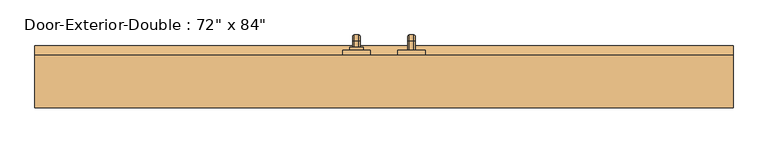
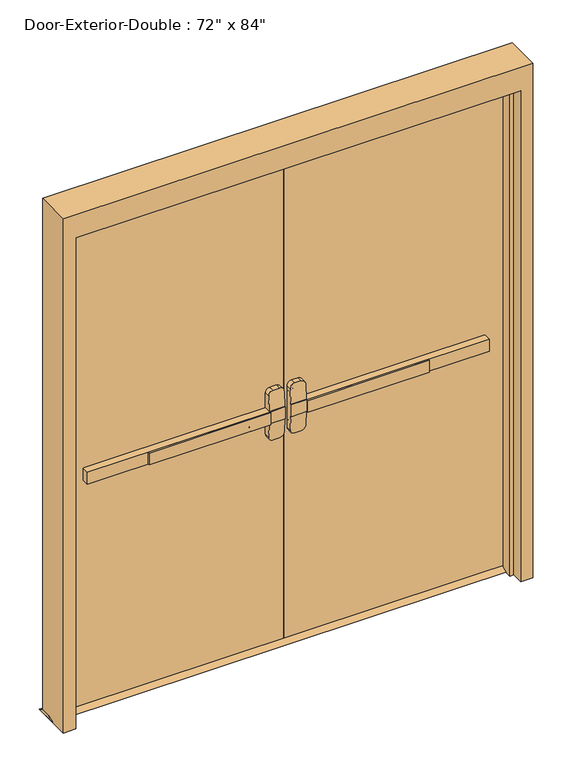
"""IFC4 building model written with IfcOpenShell, lengths in millimetres: door geometry."""

from ifc_helpers import new_model, si_unit, point, frame, frame_2d, origin, place, context, project, spatial, polyline, circle_curve, ellipse_curve, trimmed, segment, composite_curve, outline, extrude, faceted_brep, source, transform, mapped, element, save
from ifc_brep_helpers import plane_surface, cylinder_surface, revolved_surface, advanced_brep


def door_9c6f9228(model_context):
    return source(origin(), model_context, "Body", "SolidModel", [
        extrude(outline(polyline([(-575.7333333, -3.175), (-575.7333333, 3.175), (-76.2, 3.175), (-76.2, -3.175), (-575.7333333, -3.175)])), frame((0.0, 0.0, 990.6), z_axis=(0.0, 0.0, 1.0), x_axis=(1.0, 0.0, 0.0)), (0.0, 0.0, 1.0), 50.8),
        advanced_brep(
        [(-12.7, 3.175, 1041.4), (-76.2, 3.175, 1041.4), (-825.5, 3.175, 1041.4), (-825.5, 3.175, 990.6), (-76.2, 3.175, 990.6), (-12.7, 3.175, 990.6), (-825.5, 34.925, 1041.4), (-76.2, 34.925, 1041.4), (-76.2, 34.925, 1104.9), (-57.15, 34.925, 1123.95), (-31.75, 34.925, 1123.95), (-12.7, 34.925, 1104.9), (-12.7, 34.925, 927.1), (-31.75, 34.925, 908.05), (-57.15, 34.925, 908.05), (-76.2, 34.925, 927.1), (-76.2, 34.925, 990.6), (-825.5, 34.925, 990.6), (-12.7, 6.3502467, 1041.4), (-76.2, 6.3502467, 1041.4), (-12.7, 6.3502467, 990.6), (-12.7, 11.3604269, 927.1), (-12.7, 11.3604269, 1104.9), (-76.2, 6.3502467, 990.6), (-76.2, 11.3604269, 1104.9), (-76.2, 11.3604269, 927.1), (-57.15, 12.863481, 1123.95), (-31.75, 12.863481, 1123.95), (-31.75, 12.863481, 908.05), (-57.15, 12.863481, 908.05)],
        [
            (0, 1),
            (1, 2),
            (2, 3),
            (3, 4),
            (4, 5),
            (5, 0),
            (6, 7),
            (7, 8),
            (8, 9, circle_curve(frame((-57.15, 34.925, 1104.9), z_axis=(0.0, 1.0, 0.0), x_axis=(-1.0, 0.0, 0.0)), 19.05)),
            (9, 10),
            (10, 11, circle_curve(frame((-31.75, 34.925, 1104.9), z_axis=(0.0, 1.0, 0.0), x_axis=(-1.0, 0.0, 0.0)), 19.05)),
            (11, 12),
            (12, 13, circle_curve(frame((-31.75, 34.925, 927.1), z_axis=(0.0, 1.0, 0.0), x_axis=(-1.0, 0.0, 0.0)), 19.05)),
            (13, 14),
            (14, 15, circle_curve(frame((-57.15, 34.925, 927.1), z_axis=(0.0, 1.0, 0.0), x_axis=(-1.0, 0.0, 0.0)), 19.05)),
            (15, 16),
            (16, 17),
            (17, 6),
            (0, 18),
            (18, 19),
            (19, 7),
            (6, 2),
            (5, 20),
            (20, 21),
            (21, 12),
            (11, 22),
            (22, 18),
            (16, 23),
            (23, 20),
            (3, 17),
            (19, 24),
            (24, 8),
            (15, 25),
            (25, 23),
            (9, 26),
            (26, 27),
            (27, 10),
            (13, 28),
            (28, 29),
            (29, 14),
            (29, 25, ellipse_curve(frame((-57.15, 11.3604269, 927.1), z_axis=(0.0, 0.9969018152893365, 0.07865602756830282), x_axis=(0.0, -0.07865602756830208, 0.9969018152893365)), 19.1092038, 19.05)),
            (24, 26, ellipse_curve(frame((-57.15, 11.3604269, 1104.9), z_axis=(0.0, 0.9969018152893376, -0.07865602756828934), x_axis=(0.0, -0.078656027568288, -0.9969018152893377)), 19.1092038, 19.05)),
            (27, 22, ellipse_curve(frame((-31.75, 11.3604269, 1104.9), z_axis=(0.0, 0.9969018152893376, -0.07865602756828934), x_axis=(0.0, -0.078656027568288, -0.9969018152893377)), 19.1092038, 19.05)),
            (21, 28, ellipse_curve(frame((-31.75, 11.3604269, 927.1), z_axis=(0.0, 0.9969018152893365, 0.07865602756830282), x_axis=(0.0, -0.07865602756830208, 0.9969018152893365)), 19.1092038, 19.05)),
        ],
        [
            plane_surface(frame((-12.7, 3.175, 1041.4), z_axis=(0.0, -1.0, 0.0), x_axis=(1.0, 0.0, 0.0))),
            plane_surface(frame((-12.7, 34.925, 1041.4), z_axis=(0.0, 1.0, 0.0), x_axis=(-1.0, 0.0, 0.0))),
            plane_surface(frame((-825.5, 3.175, 1041.4), z_axis=(0.0, 0.0, 1.0), x_axis=(0.0, 1.0, 0.0))),
            plane_surface(frame((-12.7, 3.175, 1041.4), z_axis=(1.0, 0.0, 0.0), x_axis=(0.0, 1.0, 0.0))),
            plane_surface(frame((-12.7, 3.175, 990.6), z_axis=(0.0, 0.0, -1.0), x_axis=(0.0, 1.0, 0.0))),
            plane_surface(frame((-825.5, 3.175, 990.6), z_axis=(-1.0, 0.0, 0.0), x_axis=(0.0, 1.0, 0.0))),
            plane_surface(frame((-76.2, 6.3502467, 927.1), z_axis=(-1.0, 0.0, 0.0), x_axis=(0.0, 1.0, 0.0))),
            plane_surface(frame((-57.15, 6.3502467, 1123.95), z_axis=(0.0, 0.0, 1.0), x_axis=(0.0, 1.0, 0.0))),
            plane_surface(frame((-31.75, 6.3502467, 908.05), z_axis=(0.0, 0.0, -1.0), x_axis=(0.0, 1.0, 0.0))),
            cylinder_surface(frame((-57.15, 34.925, 927.1), z_axis=(0.0, -1.0, 0.0), x_axis=(-1.0, 0.0, 0.0)), 19.05),
            cylinder_surface(frame((-57.15, 34.925, 1104.9), z_axis=(0.0, -1.0, 0.0), x_axis=(-1.0, 0.0, 0.0)), 19.05),
            cylinder_surface(frame((-31.75, 34.925, 1104.9), z_axis=(0.0, -1.0, 0.0), x_axis=(-1.0, 0.0, 0.0)), 19.05),
            cylinder_surface(frame((-31.75, 34.925, 927.1), z_axis=(0.0, -1.0, 0.0), x_axis=(-1.0, 0.0, 0.0)), 19.05),
            plane_surface(frame((-76.2, 6.3502467, 1041.4), z_axis=(0.0, -0.9969018152893376, 0.07865602756828934), x_axis=(1.0, 0.0, 0.0))),
            plane_surface(frame((-76.2, 12.863481, 908.05), z_axis=(0.0, -0.9969018152893365, -0.07865602756830282), x_axis=(1.0, 0.0, 0.0))),
        ],
        [
            (0, [[1, 2, 3, 4, 5, 6]]),
            (1, [[7, 8, 9, 10, 11, 12, 13, 14, 15, 16, 17, 18]]),
            (2, [[-2, -1, 19, 20, 21, -7, 22]]),
            (3, [[23, 24, 25, -12, 26, 27, -19, -6]]),
            (4, [[-17, 28, 29, -23, -5, -4, 30]]),
            (5, [[-22, -18, -30, -3]]),
            (6, [[-21, 31, 32, -8]]),
            (6, [[33, 34, -28, -16]]),
            (7, [[35, 36, 37, -10]]),
            (8, [[38, 39, 40, -14]]),
            (9, [[-40, 41, -33, -15]]),
            (10, [[-32, 42, -35, -9]]),
            (11, [[-37, 43, -26, -11]]),
            (12, [[-25, 44, -38, -13]]),
            (13, [[-27, -43, -36, -42, -31, -20]]),
            (14, [[-29, -34, -41, -39, -44, -24]]),
        ],
    ),
        extrude(outline(polyline([(79.375, 12.7), (104.775, 0.0), (9.525, 0.0), (34.925, 12.7), (79.375, 12.7)])), frame((-965.2, 0.0, 0.0), z_axis=(1.0, 0.0, 0.0), x_axis=(0.0, 1.0, 0.0)), (0.0, 0.0, 1.0), 1930.4),
        extrude(outline(polyline([(575.7333333, -3.175), (76.2, -3.175), (76.2, 3.175), (575.7333333, 3.175), (575.7333333, -3.175)])), frame((0.0, 0.0, 990.6), z_axis=(0.0, 0.0, 1.0), x_axis=(1.0, 0.0, 0.0)), (0.0, 0.0, 1.0), 50.8),
        advanced_brep(
        [(12.7, 3.175, 1041.4), (12.7, 3.175, 990.6), (76.2, 3.175, 990.6), (825.5, 3.175, 990.6), (825.5, 3.175, 1041.4), (76.2, 3.175, 1041.4), (825.5, 34.925, 1041.4), (825.5, 34.925, 990.6), (76.2, 34.925, 990.6), (76.2, 34.925, 927.1), (57.15, 34.925, 908.05), (31.75, 34.925, 908.05), (12.7, 34.925, 927.1), (12.7, 34.925, 1104.9), (31.75, 34.925, 1123.95), (57.15, 34.925, 1123.95), (76.2, 34.925, 1104.9), (76.2, 34.925, 1041.4), (76.2, 6.3502467, 1041.4), (12.7, 6.3502467, 1041.4), (12.7, 11.3604269, 1104.9), (12.7, 11.3604269, 927.1), (12.7, 6.3502467, 990.6), (76.2, 6.3502467, 990.6), (76.2, 11.3604269, 927.1), (76.2, 11.3604269, 1104.9), (31.75, 12.863481, 1123.95), (57.15, 12.863481, 1123.95), (57.15, 12.863481, 908.05), (31.75, 12.863481, 908.05)],
        [
            (0, 1),
            (1, 2),
            (2, 3),
            (3, 4),
            (4, 5),
            (5, 0),
            (6, 7),
            (7, 8),
            (8, 9),
            (9, 10, circle_curve(frame((57.15, 34.925, 927.1), z_axis=(0.0, 1.0, 0.0), x_axis=(1.0, 0.0, 0.0)), 19.05)),
            (10, 11),
            (11, 12, circle_curve(frame((31.75, 34.925, 927.1), z_axis=(0.0, 1.0, 0.0), x_axis=(1.0, 0.0, 0.0)), 19.05)),
            (12, 13),
            (13, 14, circle_curve(frame((31.75, 34.925, 1104.9), z_axis=(0.0, 1.0, 0.0), x_axis=(1.0, 0.0, 0.0)), 19.05)),
            (14, 15),
            (15, 16, circle_curve(frame((57.15, 34.925, 1104.9), z_axis=(0.0, 1.0, 0.0), x_axis=(1.0, 0.0, 0.0)), 19.05)),
            (16, 17),
            (17, 6),
            (4, 6),
            (17, 18),
            (18, 19),
            (19, 0),
            (19, 20),
            (20, 13),
            (12, 21),
            (21, 22),
            (22, 1),
            (7, 3),
            (22, 23),
            (23, 8),
            (23, 24),
            (24, 9),
            (16, 25),
            (25, 18),
            (14, 26),
            (26, 27),
            (27, 15),
            (10, 28),
            (28, 29),
            (29, 11),
            (24, 28, ellipse_curve(frame((57.15, 11.3604269, 927.1), z_axis=(0.0, 0.9969018152893365, 0.07865602756830282), x_axis=(0.0, -0.07865602756830208, 0.9969018152893365)), 19.1092038, 19.05)),
            (27, 25, ellipse_curve(frame((57.15, 11.3604269, 1104.9), z_axis=(0.0, 0.9969018152893376, -0.07865602756828934), x_axis=(0.0, -0.078656027568288, -0.9969018152893377)), 19.1092038, 19.05)),
            (20, 26, ellipse_curve(frame((31.75, 11.3604269, 1104.9), z_axis=(0.0, 0.9969018152893376, -0.07865602756828934), x_axis=(0.0, -0.078656027568288, -0.9969018152893377)), 19.1092038, 19.05)),
            (29, 21, ellipse_curve(frame((31.75, 11.3604269, 927.1), z_axis=(0.0, 0.9969018152893365, 0.07865602756830282), x_axis=(0.0, -0.07865602756830208, 0.9969018152893365)), 19.1092038, 19.05)),
        ],
        [
            plane_surface(frame((12.7, 3.175, 1041.4), z_axis=(0.0, -1.0, 0.0), x_axis=(-1.0, 0.0, 0.0))),
            plane_surface(frame((12.7, 34.925, 1041.4), z_axis=(0.0, 1.0, 0.0), x_axis=(1.0, 0.0, 0.0))),
            plane_surface(frame((825.5, 3.175, 1041.4), z_axis=(0.0, 0.0, 1.0), x_axis=(0.0, 1.0, 0.0))),
            plane_surface(frame((12.7, 3.175, 1041.4), z_axis=(-1.0, 0.0, 0.0), x_axis=(0.0, 1.0, 0.0))),
            plane_surface(frame((12.7, 3.175, 990.6), z_axis=(0.0, 0.0, -1.0), x_axis=(0.0, 1.0, 0.0))),
            plane_surface(frame((825.5, 3.175, 990.6), z_axis=(1.0, 0.0, 0.0), x_axis=(0.0, 1.0, 0.0))),
            plane_surface(frame((76.2, 6.3502467, 927.1), z_axis=(1.0, 0.0, 0.0), x_axis=(0.0, 1.0, 0.0))),
            plane_surface(frame((57.15, 6.3502467, 1123.95), z_axis=(0.0, 0.0, 1.0), x_axis=(0.0, 1.0, 0.0))),
            plane_surface(frame((31.75, 6.3502467, 908.05), z_axis=(0.0, 0.0, -1.0), x_axis=(0.0, 1.0, 0.0))),
            cylinder_surface(frame((57.15, 34.925, 927.1), z_axis=(0.0, -1.0, 0.0), x_axis=(1.0, 0.0, 0.0)), 19.05),
            cylinder_surface(frame((57.15, 34.925, 1104.9), z_axis=(0.0, -1.0, 0.0), x_axis=(1.0, 0.0, 0.0)), 19.05),
            cylinder_surface(frame((31.75, 34.925, 1104.9), z_axis=(0.0, -1.0, 0.0), x_axis=(1.0, 0.0, 0.0)), 19.05),
            cylinder_surface(frame((31.75, 34.925, 927.1), z_axis=(0.0, -1.0, 0.0), x_axis=(1.0, 0.0, 0.0)), 19.05),
            plane_surface(frame((76.2, 6.3502467, 1041.4), z_axis=(0.0, -0.9969018152893376, 0.07865602756828934), x_axis=(-1.0, 0.0, 0.0))),
            plane_surface(frame((76.2, 12.863481, 908.05), z_axis=(0.0, -0.9969018152893365, -0.07865602756830282), x_axis=(-1.0, 0.0, 0.0))),
        ],
        [
            (0, [[1, 2, 3, 4, 5, 6]]),
            (1, [[7, 8, 9, 10, 11, 12, 13, 14, 15, 16, 17, 18]]),
            (2, [[19, -18, 20, 21, 22, -6, -5]]),
            (3, [[-1, -22, 23, 24, -13, 25, 26, 27]]),
            (4, [[28, -3, -2, -27, 29, 30, -8]]),
            (5, [[-4, -28, -7, -19]]),
            (6, [[-9, -30, 31, 32]]),
            (6, [[-17, 33, 34, -20]]),
            (7, [[-15, 35, 36, 37]]),
            (8, [[-11, 38, 39, 40]]),
            (9, [[-10, -32, 41, -38]]),
            (10, [[-16, -37, 42, -33]]),
            (11, [[-14, -24, 43, -35]]),
            (12, [[-12, -40, 44, -25]]),
            (13, [[-21, -34, -42, -36, -43, -23]]),
            (14, [[-26, -44, -39, -41, -31, -29]]),
        ],
    ),
        advanced_brep(
        [(66.2, 92.075, 1017.190625), (66.2, 92.075, 1014.809375), (69.771875, 92.075, 1011.2375), (82.6284594, 92.075, 1011.2375), (86.2, 92.075, 1014.8090406), (86.2, 92.075, 1017.190625), (82.628125, 92.075, 1020.7625), (69.771875, 92.075, 1020.7625), (66.2, 92.075, 887.809375), (69.771875, 92.075, 884.2375), (82.628125, 92.075, 884.2375), (86.2, 92.075, 887.809375), (86.2, 92.075, 890.1909594), (82.6284594, 92.075, 893.7625), (69.771875, 92.075, 893.7625), (66.2, 92.075, 890.190625), (66.2, 117.475, 1017.190625), (66.2, 131.365625, 1003.3), (66.2, 131.365625, 901.7), (66.2, 117.475, 887.809375), (66.2, 117.475, 890.190625), (66.2, 128.984375, 901.7), (66.2, 128.984375, 1003.3), (66.2, 117.475, 1014.809375), (69.771875, 117.475, 1011.2375), (82.6284594, 117.475, 1011.2375), (86.2, 117.475, 1014.8090406), (86.2, 128.9840406, 1003.3), (86.2, 128.9840406, 901.7), (86.2, 117.475, 890.1909594), (86.2, 117.475, 887.809375), (86.2, 131.365625, 901.7), (86.2, 131.365625, 1003.3), (86.2, 117.475, 1017.190625), (82.628125, 117.475, 1020.7625), (69.771875, 117.475, 1020.7625), (69.771875, 125.4125, 1003.3), (82.6284594, 125.4125, 1003.3), (82.628125, 134.9375, 1003.3), (69.771875, 134.9375, 1003.3), (69.771875, 125.4125, 901.7), (82.6284594, 125.4125, 901.7), (82.628125, 134.9375, 901.7), (69.771875, 134.9375, 901.7), (69.771875, 117.475, 893.7625), (82.6284594, 117.475, 893.7625), (82.628125, 117.475, 884.2375), (69.771875, 117.475, 884.2375)],
        [
            (0, 1),
            (1, 2, circle_curve(frame((69.771875, 92.075, 1014.809375), z_axis=(0.0, -1.0, 0.0), x_axis=(0.0, 0.0, 1.0)), 3.571875)),
            (2, 3),
            (3, 4, circle_curve(frame((82.6284594, 92.075, 1014.8090406), z_axis=(0.0, -1.0, 0.0), x_axis=(0.0, 0.0, 1.0)), 3.5715406)),
            (4, 5),
            (5, 6, circle_curve(frame((82.628125, 92.075, 1017.190625), z_axis=(0.0, -1.0, 0.0), x_axis=(0.0, 0.0, 1.0)), 3.571875)),
            (6, 7),
            (7, 0, circle_curve(frame((69.771875, 92.075, 1017.190625), z_axis=(0.0, -1.0, 0.0), x_axis=(0.0, 0.0, 1.0)), 3.571875)),
            (8, 9, circle_curve(frame((69.771875, 92.075, 887.809375), z_axis=(0.0, -1.0, 0.0), x_axis=(0.0, 0.0, -1.0)), 3.571875)),
            (9, 10),
            (10, 11, circle_curve(frame((82.628125, 92.075, 887.809375), z_axis=(0.0, -1.0, 0.0), x_axis=(0.0, 0.0, -1.0)), 3.571875)),
            (11, 12),
            (12, 13, circle_curve(frame((82.6284594, 92.075, 890.1909594), z_axis=(0.0, -1.0, 0.0), x_axis=(0.0, 0.0, -1.0)), 3.5715406)),
            (13, 14),
            (14, 15, circle_curve(frame((69.771875, 92.075, 890.190625), z_axis=(0.0, -1.0, 0.0), x_axis=(0.0, 0.0, -1.0)), 3.571875)),
            (15, 8),
            (0, 16),
            (16, 17, circle_curve(frame((66.2, 117.475, 1003.3), z_axis=(-1.0, 0.0, 0.0), x_axis=(0.0, 0.0, 1.0)), 13.890625)),
            (17, 18),
            (18, 19, circle_curve(frame((66.2, 117.475, 901.7), z_axis=(-1.0, 0.0, 0.0), x_axis=(0.0, 1.0, 0.0)), 13.890625)),
            (19, 8),
            (15, 20),
            (20, 21, circle_curve(frame((66.2, 117.475, 901.7), z_axis=(1.0, 0.0, 0.0), x_axis=(0.0, 1.0, 0.0)), 11.509375)),
            (21, 22),
            (22, 23, circle_curve(frame((66.2, 117.475, 1003.3), z_axis=(1.0, 0.0, 0.0), x_axis=(0.0, 0.0, 1.0)), 11.509375)),
            (23, 1),
            (23, 24, circle_curve(frame((69.771875, 117.475, 1014.809375), z_axis=(0.0, -1.0, 0.0), x_axis=(0.0, 0.0, 1.0)), 3.571875)),
            (24, 2),
            (24, 25),
            (25, 3),
            (25, 26, circle_curve(frame((82.6284594, 117.475, 1014.8090406), z_axis=(0.0, -1.0, 0.0), x_axis=(0.0, 0.0, 1.0)), 3.5715406)),
            (26, 4),
            (26, 27, circle_curve(frame((86.2, 117.475, 1003.3), z_axis=(-1.0, 0.0, 0.0), x_axis=(0.0, 0.0, 1.0)), 11.5090406)),
            (27, 28),
            (28, 29, circle_curve(frame((86.2, 117.475, 901.7), z_axis=(-1.0, 0.0, 0.0), x_axis=(0.0, 1.0, 0.0)), 11.5090406)),
            (29, 12),
            (11, 30),
            (30, 31, circle_curve(frame((86.2, 117.475, 901.7), z_axis=(1.0, 0.0, 0.0), x_axis=(0.0, 1.0, 0.0)), 13.890625)),
            (31, 32),
            (32, 33, circle_curve(frame((86.2, 117.475, 1003.3), z_axis=(1.0, 0.0, 0.0), x_axis=(0.0, 0.0, 1.0)), 13.890625)),
            (33, 5),
            (33, 34, circle_curve(frame((82.628125, 117.475, 1017.190625), z_axis=(0.0, -1.0, 0.0), x_axis=(0.0, 0.0, 1.0)), 3.571875)),
            (34, 6),
            (34, 35),
            (35, 7),
            (35, 16, circle_curve(frame((69.771875, 117.475, 1017.190625), z_axis=(0.0, -1.0, 0.0), x_axis=(0.0, 0.0, 1.0)), 3.571875)),
            (36, 24, circle_curve(frame((69.771875, 117.475, 1003.3), z_axis=(1.0, 0.0, 0.0), x_axis=(0.0, 0.0, 1.0)), 7.9375)),
            (22, 36, circle_curve(frame((69.771875, 128.984375, 1003.3), z_axis=(0.0, 0.0, 1.0), x_axis=(0.0, 1.0, 0.0)), 3.571875)),
            (37, 25, circle_curve(frame((82.6284594, 117.475, 1003.3), z_axis=(1.0, 0.0, 0.0), x_axis=(0.0, 0.0, 1.0)), 7.9375)),
            (36, 37),
            (37, 27, circle_curve(frame((82.6284594, 128.9840406, 1003.3), z_axis=(0.0, 0.0, 1.0), x_axis=(0.0, 1.0, 0.0)), 3.5715406)),
            (38, 34, circle_curve(frame((82.628125, 117.475, 1003.3), z_axis=(1.0, 0.0, 0.0), x_axis=(0.0, 0.0, 1.0)), 17.4625)),
            (32, 38, circle_curve(frame((82.628125, 131.365625, 1003.3), z_axis=(0.0, 0.0, 1.0), x_axis=(0.0, 1.0, 0.0)), 3.571875)),
            (39, 35, circle_curve(frame((69.771875, 117.475, 1003.3), z_axis=(1.0, 0.0, 0.0), x_axis=(0.0, 0.0, 1.0)), 17.4625)),
            (38, 39),
            (39, 17, circle_curve(frame((69.771875, 131.365625, 1003.3), z_axis=(0.0, 0.0, 1.0), x_axis=(0.0, 1.0, 0.0)), 3.571875)),
            (21, 40, circle_curve(frame((69.771875, 128.984375, 901.7), z_axis=(0.0, 0.0, 1.0), x_axis=(0.0, 1.0, 0.0)), 3.571875)),
            (40, 36),
            (40, 41),
            (41, 37),
            (41, 28, circle_curve(frame((82.6284594, 128.9840406, 901.7), z_axis=(0.0, 0.0, 1.0), x_axis=(0.0, 1.0, 0.0)), 3.5715406)),
            (31, 42, circle_curve(frame((82.628125, 131.365625, 901.7), z_axis=(0.0, 0.0, 1.0), x_axis=(0.0, 1.0, 0.0)), 3.571875)),
            (42, 38),
            (42, 43),
            (43, 39),
            (43, 18, circle_curve(frame((69.771875, 131.365625, 901.7), z_axis=(0.0, 0.0, 1.0), x_axis=(0.0, 1.0, 0.0)), 3.571875)),
            (44, 40, circle_curve(frame((69.771875, 117.475, 901.7), z_axis=(1.0, 0.0, 0.0), x_axis=(0.0, 1.0, 0.0)), 7.9375)),
            (20, 44, circle_curve(frame((69.771875, 117.475, 890.190625), z_axis=(0.0, 1.0, 0.0), x_axis=(0.0, 0.0, -1.0)), 3.571875)),
            (45, 41, circle_curve(frame((82.6284594, 117.475, 901.7), z_axis=(1.0, 0.0, 0.0), x_axis=(0.0, 1.0, 0.0)), 7.9375)),
            (44, 45),
            (45, 29, circle_curve(frame((82.6284594, 117.475, 890.1909594), z_axis=(0.0, 1.0, 0.0), x_axis=(0.0, 0.0, -1.0)), 3.5715406)),
            (46, 42, circle_curve(frame((82.628125, 117.475, 901.7), z_axis=(1.0, 0.0, 0.0), x_axis=(0.0, 1.0, 0.0)), 17.4625)),
            (30, 46, circle_curve(frame((82.628125, 117.475, 887.809375), z_axis=(0.0, 1.0, 0.0), x_axis=(0.0, 0.0, -1.0)), 3.571875)),
            (47, 43, circle_curve(frame((69.771875, 117.475, 901.7), z_axis=(1.0, 0.0, 0.0), x_axis=(0.0, 1.0, 0.0)), 17.4625)),
            (46, 47),
            (47, 19, circle_curve(frame((69.771875, 117.475, 887.809375), z_axis=(0.0, 1.0, 0.0), x_axis=(0.0, 0.0, -1.0)), 3.571875)),
            (14, 44),
            (13, 45),
            (10, 46),
            (9, 47),
        ],
        [
            plane_surface(frame((76.2, 92.075, 1016.0), z_axis=(0.0, -1.0, 0.0), x_axis=(1.0, 0.0, 0.0))),
            plane_surface(frame((76.2, 92.075, 889.0), z_axis=(0.0, -1.0, 0.0), x_axis=(1.0, 0.0, 0.0))),
            plane_surface(frame((66.2, 92.075, 1017.190625), z_axis=(-1.0, 0.0, 0.0), x_axis=(0.0, 1.0, 0.0))),
            cylinder_surface(frame((69.771875, 92.075, 1014.809375), z_axis=(0.0, -1.0, 0.0), x_axis=(0.0, 0.0, 1.0)), 3.571875),
            plane_surface(frame((69.771875, 92.075, 1011.2375), z_axis=(0.0, 0.0, -1.0), x_axis=(0.0, 1.0, 0.0))),
            cylinder_surface(frame((82.6284594, 92.075, 1014.8090406), z_axis=(0.0, -1.0, 0.0), x_axis=(0.0, 0.0, 1.0)), 3.5715406),
            plane_surface(frame((86.2, 92.075, 1014.8090406), z_axis=(1.0, 0.0, 0.0), x_axis=(0.0, 1.0, 0.0))),
            cylinder_surface(frame((82.628125, 92.075, 1017.190625), z_axis=(0.0, -1.0, 0.0), x_axis=(0.0, 0.0, 1.0)), 3.571875),
            plane_surface(frame((82.628125, 92.075, 1020.7625), z_axis=(0.0, 0.0, 1.0), x_axis=(0.0, 1.0, 0.0))),
            cylinder_surface(frame((69.771875, 92.075, 1017.190625), z_axis=(0.0, -1.0, 0.0), x_axis=(0.0, 0.0, 1.0)), 3.571875),
            revolved_surface(trimmed(ellipse_curve(frame((69.771875, 117.475, 1014.809375), z_axis=(0.0, -1.0, 0.0), x_axis=(0.0, 0.0, 1.0)), 3.571875, 3.571875), [point((66.2, 117.475, 1014.809375))], [point((69.771875, 117.475, 1011.2375))], True, "CARTESIAN"), (76.2, 117.475, 1003.3), (-1.0, 0.0, 0.0)),
            revolved_surface(polyline([(69.771875, 117.475, 1011.2375), (82.6284594, 117.475, 1011.2375)]), (76.2, 117.475, 1003.3), (-1.0, 0.0, 0.0)),
            revolved_surface(trimmed(ellipse_curve(frame((82.6284594, 117.475, 1014.8090406), z_axis=(0.0, -1.0, 0.0), x_axis=(0.0, 0.0, 1.0)), 3.5715406, 3.5715406), [point((82.6284594, 117.475, 1011.2375))], [point((86.2, 117.475, 1014.8090406))], True, "CARTESIAN"), (76.2, 117.475, 1003.3), (-1.0, 0.0, 0.0)),
            revolved_surface(trimmed(ellipse_curve(frame((82.628125, 117.475, 1017.190625), z_axis=(0.0, -1.0, 0.0), x_axis=(0.0, 0.0, 1.0)), 3.571875, 3.571875), [point((86.2, 117.475, 1017.190625))], [point((82.628125, 117.475, 1020.7625))], True, "CARTESIAN"), (76.2, 117.475, 1003.3), (-1.0, 0.0, 0.0)),
            cylinder_surface(frame((76.2, 117.475, 1003.3), z_axis=(-1.0, 0.0, 0.0), x_axis=(0.0, 0.0, 1.0)), 17.4625),
            revolved_surface(trimmed(ellipse_curve(frame((69.771875, 117.475, 1017.190625), z_axis=(0.0, -1.0, 0.0), x_axis=(0.0, 0.0, 1.0)), 3.571875, 3.571875), [point((69.771875, 117.475, 1020.7625))], [point((66.2, 117.475, 1017.190625))], True, "CARTESIAN"), (76.2, 117.475, 1003.3), (-1.0, 0.0, 0.0)),
            cylinder_surface(frame((69.771875, 128.984375, 1003.3), z_axis=(0.0, 0.0, 1.0), x_axis=(0.0, 1.0, 0.0)), 3.571875),
            plane_surface(frame((69.771875, 125.4125, 1003.3), z_axis=(0.0, -1.0, 0.0), x_axis=(0.0, 0.0, -1.0))),
            cylinder_surface(frame((82.6284594, 128.9840406, 1003.3), z_axis=(0.0, 0.0, 1.0), x_axis=(0.0, 1.0, 0.0)), 3.5715406),
            cylinder_surface(frame((82.628125, 131.365625, 1003.3), z_axis=(0.0, 0.0, 1.0), x_axis=(0.0, 1.0, 0.0)), 3.571875),
            plane_surface(frame((82.628125, 134.9375, 1003.3), z_axis=(0.0, 1.0, 0.0), x_axis=(0.0, 0.0, -1.0))),
            cylinder_surface(frame((69.771875, 131.365625, 1003.3), z_axis=(0.0, 0.0, 1.0), x_axis=(0.0, 1.0, 0.0)), 3.571875),
            revolved_surface(trimmed(ellipse_curve(frame((69.771875, 128.984375, 901.7), z_axis=(0.0, 0.0, 1.0), x_axis=(0.0, 1.0, 0.0)), 3.571875, 3.571875), [point((66.2, 128.984375, 901.7))], [point((69.771875, 125.4125, 901.7))], True, "CARTESIAN"), (76.2, 117.475, 901.7), (-1.0, 0.0, 0.0)),
            revolved_surface(polyline([(69.771875, 125.4125, 901.7), (82.6284594, 125.4125, 901.7)]), (76.2, 117.475, 901.7), (-1.0, 0.0, 0.0)),
            revolved_surface(trimmed(ellipse_curve(frame((82.6284594, 128.9840406, 901.7), z_axis=(0.0, 0.0, 1.0), x_axis=(0.0, 1.0, 0.0)), 3.5715406, 3.5715406), [point((82.6284594, 125.4125, 901.7))], [point((86.2, 128.9840406, 901.7))], True, "CARTESIAN"), (76.2, 117.475, 901.7), (-1.0, 0.0, 0.0)),
            revolved_surface(trimmed(ellipse_curve(frame((82.628125, 131.365625, 901.7), z_axis=(0.0, 0.0, 1.0), x_axis=(0.0, 1.0, 0.0)), 3.571875, 3.571875), [point((86.2, 131.365625, 901.7))], [point((82.628125, 134.9375, 901.7))], True, "CARTESIAN"), (76.2, 117.475, 901.7), (-1.0, 0.0, 0.0)),
            cylinder_surface(frame((76.2, 117.475, 901.7), z_axis=(-1.0, 0.0, 0.0), x_axis=(0.0, 1.0, 0.0)), 17.4625),
            revolved_surface(trimmed(ellipse_curve(frame((69.771875, 131.365625, 901.7), z_axis=(0.0, 0.0, 1.0), x_axis=(0.0, 1.0, 0.0)), 3.571875, 3.571875), [point((69.771875, 134.9375, 901.7))], [point((66.2, 131.365625, 901.7))], True, "CARTESIAN"), (76.2, 117.475, 901.7), (-1.0, 0.0, 0.0)),
            cylinder_surface(frame((69.771875, 117.475, 890.190625), z_axis=(0.0, 1.0, 0.0), x_axis=(0.0, 0.0, -1.0)), 3.571875),
            plane_surface(frame((69.771875, 117.475, 893.7625), z_axis=(0.0, 0.0, 1.0), x_axis=(0.0, -1.0, 0.0))),
            cylinder_surface(frame((82.6284594, 117.475, 890.1909594), z_axis=(0.0, 1.0, 0.0), x_axis=(0.0, 0.0, -1.0)), 3.5715406),
            cylinder_surface(frame((82.628125, 117.475, 887.809375), z_axis=(0.0, 1.0, 0.0), x_axis=(0.0, 0.0, -1.0)), 3.571875),
            plane_surface(frame((82.628125, 117.475, 884.2375), z_axis=(0.0, 0.0, -1.0), x_axis=(0.0, -1.0, 0.0))),
            cylinder_surface(frame((69.771875, 117.475, 887.809375), z_axis=(0.0, 1.0, 0.0), x_axis=(0.0, 0.0, -1.0)), 3.571875),
        ],
        [
            (0, [[1, 2, 3, 4, 5, 6, 7, 8]]),
            (1, [[9, 10, 11, 12, 13, 14, 15, 16]]),
            (2, [[-1, 17, 18, 19, 20, 21, -16, 22, 23, 24, 25, 26]]),
            (3, [[-2, -26, 27, 28]]),
            (4, [[-3, -28, 29, 30]]),
            (5, [[-4, -30, 31, 32]]),
            (6, [[-5, -32, 33, 34, 35, 36, -12, 37, 38, 39, 40, 41]]),
            (7, [[-6, -41, 42, 43]]),
            (8, [[-7, -43, 44, 45]]),
            (9, [[-8, -45, 46, -17]]),
            (10, [[47, -27, -25, 48]]),
            (11, [[49, -29, -47, 50]]),
            (12, [[-33, -31, -49, 51]]),
            (13, [[52, -42, -40, 53]]),
            (14, [[54, -44, -52, 55]]),
            (15, [[-18, -46, -54, 56]]),
            (16, [[-48, -24, 57, 58]]),
            (17, [[-50, -58, 59, 60]]),
            (18, [[-51, -60, 61, -34]]),
            (19, [[-53, -39, 62, 63]]),
            (20, [[-55, -63, 64, 65]]),
            (21, [[-56, -65, 66, -19]]),
            (22, [[67, -57, -23, 68]]),
            (23, [[69, -59, -67, 70]]),
            (24, [[-35, -61, -69, 71]]),
            (25, [[72, -62, -38, 73]]),
            (26, [[74, -64, -72, 75]]),
            (27, [[-20, -66, -74, 76]]),
            (28, [[-68, -22, -15, 77]]),
            (29, [[-70, -77, -14, 78]]),
            (30, [[-71, -78, -13, -36]]),
            (31, [[-73, -37, -11, 79]]),
            (32, [[-75, -79, -10, 80]]),
            (33, [[-76, -80, -9, -21]]),
        ],
    ),
        extrude(outline(composite_curve([segment(trimmed(circle_curve(frame_2d((1113.0338574, 76.2)), 89.3016225), [point((1193.8, 114.3))], [point((1193.8, 38.1))], False, "CARTESIAN"), True, "CONTINUOUS"), segment(polyline([(1193.8, 38.1), (838.2, 38.1)]), True, "CONTINUOUS"), segment(trimmed(circle_curve(frame_2d((918.9661426, 76.2)), 89.3016225), [point((838.2, 38.1))], [point((838.2, 114.3))], False, "CARTESIAN"), True, "CONTINUOUS"), segment(polyline([(838.2, 114.3), (1193.8, 114.3)]), True, "CONTINUOUS")], self_intersect=False)), frame((0.0, 79.375, 0.0), z_axis=(0.0, 1.0, 0.0), x_axis=(0.0, 0.0, 1.0)), (0.0, 0.0, 1.0), 12.7),
        advanced_brep(
        [(-86.2, 92.075, 1017.190625), (-86.2, 92.075, 1014.809375), (-82.628125, 92.075, 1011.2375), (-69.7715406, 92.075, 1011.2375), (-66.2, 92.075, 1014.8090406), (-66.2, 92.075, 1017.190625), (-69.771875, 92.075, 1020.7625), (-82.628125, 92.075, 1020.7625), (-86.2, 92.075, 887.809375), (-82.628125, 92.075, 884.2375), (-69.771875, 92.075, 884.2375), (-66.2, 92.075, 887.809375), (-66.2, 92.075, 890.1909594), (-69.7715406, 92.075, 893.7625), (-82.628125, 92.075, 893.7625), (-86.2, 92.075, 890.190625), (-86.2, 117.475, 1017.190625), (-86.2, 131.365625, 1003.3), (-86.2, 131.365625, 901.7), (-86.2, 117.475, 887.809375), (-86.2, 117.475, 890.190625), (-86.2, 128.984375, 901.7), (-86.2, 128.984375, 1003.3), (-86.2, 117.475, 1014.809375), (-82.628125, 117.475, 1011.2375), (-69.7715406, 117.475, 1011.2375), (-66.2, 117.475, 1014.8090406), (-66.2, 128.9840406, 1003.3), (-66.2, 128.9840406, 901.7), (-66.2, 117.475, 890.1909594), (-66.2, 117.475, 887.809375), (-66.2, 131.365625, 901.7), (-66.2, 131.365625, 1003.3), (-66.2, 117.475, 1017.190625), (-69.771875, 117.475, 1020.7625), (-82.628125, 117.475, 1020.7625), (-82.628125, 125.4125, 1003.3), (-69.7715406, 125.4125, 1003.3), (-69.771875, 134.9375, 1003.3), (-82.628125, 134.9375, 1003.3), (-82.628125, 125.4125, 901.7), (-69.7715406, 125.4125, 901.7), (-69.771875, 134.9375, 901.7), (-82.628125, 134.9375, 901.7), (-82.628125, 117.475, 893.7625), (-69.7715406, 117.475, 893.7625), (-69.771875, 117.475, 884.2375), (-82.628125, 117.475, 884.2375)],
        [
            (0, 1),
            (1, 2, circle_curve(frame((-82.628125, 92.075, 1014.809375), z_axis=(0.0, -1.0, 0.0), x_axis=(0.0, 0.0, 1.0)), 3.571875)),
            (2, 3),
            (3, 4, circle_curve(frame((-69.7715406, 92.075, 1014.8090406), z_axis=(0.0, -1.0, 0.0), x_axis=(0.0, 0.0, 1.0)), 3.5715406)),
            (4, 5),
            (5, 6, circle_curve(frame((-69.771875, 92.075, 1017.190625), z_axis=(0.0, -1.0, 0.0), x_axis=(0.0, 0.0, 1.0)), 3.571875)),
            (6, 7),
            (7, 0, circle_curve(frame((-82.628125, 92.075, 1017.190625), z_axis=(0.0, -1.0, 0.0), x_axis=(0.0, 0.0, 1.0)), 3.571875)),
            (8, 9, circle_curve(frame((-82.628125, 92.075, 887.809375), z_axis=(0.0, -1.0, 0.0), x_axis=(0.0, 0.0, -1.0)), 3.571875)),
            (9, 10),
            (10, 11, circle_curve(frame((-69.771875, 92.075, 887.809375), z_axis=(0.0, -1.0, 0.0), x_axis=(0.0, 0.0, -1.0)), 3.571875)),
            (11, 12),
            (12, 13, circle_curve(frame((-69.7715406, 92.075, 890.1909594), z_axis=(0.0, -1.0, 0.0), x_axis=(0.0, 0.0, -1.0)), 3.5715406)),
            (13, 14),
            (14, 15, circle_curve(frame((-82.628125, 92.075, 890.190625), z_axis=(0.0, -1.0, 0.0), x_axis=(0.0, 0.0, -1.0)), 3.571875)),
            (15, 8),
            (0, 16),
            (16, 17, circle_curve(frame((-86.2, 117.475, 1003.3), z_axis=(-1.0, 0.0, 0.0), x_axis=(0.0, 0.0, 1.0)), 13.890625)),
            (17, 18),
            (18, 19, circle_curve(frame((-86.2, 117.475, 901.7), z_axis=(-1.0, 0.0, 0.0), x_axis=(0.0, 1.0, 0.0)), 13.890625)),
            (19, 8),
            (15, 20),
            (20, 21, circle_curve(frame((-86.2, 117.475, 901.7), z_axis=(1.0, 0.0, 0.0), x_axis=(0.0, 1.0, 0.0)), 11.509375)),
            (21, 22),
            (22, 23, circle_curve(frame((-86.2, 117.475, 1003.3), z_axis=(1.0, 0.0, 0.0), x_axis=(0.0, 0.0, 1.0)), 11.509375)),
            (23, 1),
            (23, 24, circle_curve(frame((-82.628125, 117.475, 1014.809375), z_axis=(0.0, -1.0, 0.0), x_axis=(0.0, 0.0, 1.0)), 3.571875)),
            (24, 2),
            (24, 25),
            (25, 3),
            (25, 26, circle_curve(frame((-69.7715406, 117.475, 1014.8090406), z_axis=(0.0, -1.0, 0.0), x_axis=(0.0, 0.0, 1.0)), 3.5715406)),
            (26, 4),
            (26, 27, circle_curve(frame((-66.2, 117.475, 1003.3), z_axis=(-1.0, 0.0, 0.0), x_axis=(0.0, 0.0, 1.0)), 11.5090406)),
            (27, 28),
            (28, 29, circle_curve(frame((-66.2, 117.475, 901.7), z_axis=(-1.0, 0.0, 0.0), x_axis=(0.0, 1.0, 0.0)), 11.5090406)),
            (29, 12),
            (11, 30),
            (30, 31, circle_curve(frame((-66.2, 117.475, 901.7), z_axis=(1.0, 0.0, 0.0), x_axis=(0.0, 1.0, 0.0)), 13.890625)),
            (31, 32),
            (32, 33, circle_curve(frame((-66.2, 117.475, 1003.3), z_axis=(1.0, 0.0, 0.0), x_axis=(0.0, 0.0, 1.0)), 13.890625)),
            (33, 5),
            (33, 34, circle_curve(frame((-69.771875, 117.475, 1017.190625), z_axis=(0.0, -1.0, 0.0), x_axis=(0.0, 0.0, 1.0)), 3.571875)),
            (34, 6),
            (34, 35),
            (35, 7),
            (35, 16, circle_curve(frame((-82.628125, 117.475, 1017.190625), z_axis=(0.0, -1.0, 0.0), x_axis=(0.0, 0.0, 1.0)), 3.571875)),
            (36, 24, circle_curve(frame((-82.628125, 117.475, 1003.3), z_axis=(1.0, 0.0, 0.0), x_axis=(0.0, 0.0, 1.0)), 7.9375)),
            (22, 36, circle_curve(frame((-82.628125, 128.984375, 1003.3), z_axis=(0.0, 0.0, 1.0), x_axis=(0.0, 1.0, 0.0)), 3.571875)),
            (37, 25, circle_curve(frame((-69.7715406, 117.475, 1003.3), z_axis=(1.0, 0.0, 0.0), x_axis=(0.0, 0.0, 1.0)), 7.9375)),
            (36, 37),
            (37, 27, circle_curve(frame((-69.7715406, 128.9840406, 1003.3), z_axis=(0.0, 0.0, 1.0), x_axis=(0.0, 1.0, 0.0)), 3.5715406)),
            (38, 34, circle_curve(frame((-69.771875, 117.475, 1003.3), z_axis=(1.0, 0.0, 0.0), x_axis=(0.0, 0.0, 1.0)), 17.4625)),
            (32, 38, circle_curve(frame((-69.771875, 131.365625, 1003.3), z_axis=(0.0, 0.0, 1.0), x_axis=(0.0, 1.0, 0.0)), 3.571875)),
            (39, 35, circle_curve(frame((-82.628125, 117.475, 1003.3), z_axis=(1.0, 0.0, 0.0), x_axis=(0.0, 0.0, 1.0)), 17.4625)),
            (38, 39),
            (39, 17, circle_curve(frame((-82.628125, 131.365625, 1003.3), z_axis=(0.0, 0.0, 1.0), x_axis=(0.0, 1.0, 0.0)), 3.571875)),
            (21, 40, circle_curve(frame((-82.628125, 128.984375, 901.7), z_axis=(0.0, 0.0, 1.0), x_axis=(0.0, 1.0, 0.0)), 3.571875)),
            (40, 36),
            (40, 41),
            (41, 37),
            (41, 28, circle_curve(frame((-69.7715406, 128.9840406, 901.7), z_axis=(0.0, 0.0, 1.0), x_axis=(0.0, 1.0, 0.0)), 3.5715406)),
            (31, 42, circle_curve(frame((-69.771875, 131.365625, 901.7), z_axis=(0.0, 0.0, 1.0), x_axis=(0.0, 1.0, 0.0)), 3.571875)),
            (42, 38),
            (42, 43),
            (43, 39),
            (43, 18, circle_curve(frame((-82.628125, 131.365625, 901.7), z_axis=(0.0, 0.0, 1.0), x_axis=(0.0, 1.0, 0.0)), 3.571875)),
            (44, 40, circle_curve(frame((-82.628125, 117.475, 901.7), z_axis=(1.0, 0.0, 0.0), x_axis=(0.0, 1.0, 0.0)), 7.9375)),
            (20, 44, circle_curve(frame((-82.628125, 117.475, 890.190625), z_axis=(0.0, 1.0, 0.0), x_axis=(0.0, 0.0, -1.0)), 3.571875)),
            (45, 41, circle_curve(frame((-69.7715406, 117.475, 901.7), z_axis=(1.0, 0.0, 0.0), x_axis=(0.0, 1.0, 0.0)), 7.9375)),
            (44, 45),
            (45, 29, circle_curve(frame((-69.7715406, 117.475, 890.1909594), z_axis=(0.0, 1.0, 0.0), x_axis=(0.0, 0.0, -1.0)), 3.5715406)),
            (46, 42, circle_curve(frame((-69.771875, 117.475, 901.7), z_axis=(1.0, 0.0, 0.0), x_axis=(0.0, 1.0, 0.0)), 17.4625)),
            (30, 46, circle_curve(frame((-69.771875, 117.475, 887.809375), z_axis=(0.0, 1.0, 0.0), x_axis=(0.0, 0.0, -1.0)), 3.571875)),
            (47, 43, circle_curve(frame((-82.628125, 117.475, 901.7), z_axis=(1.0, 0.0, 0.0), x_axis=(0.0, 1.0, 0.0)), 17.4625)),
            (46, 47),
            (47, 19, circle_curve(frame((-82.628125, 117.475, 887.809375), z_axis=(0.0, 1.0, 0.0), x_axis=(0.0, 0.0, -1.0)), 3.571875)),
            (14, 44),
            (13, 45),
            (10, 46),
            (9, 47),
        ],
        [
            plane_surface(frame((-76.2, 92.075, 1016.0), z_axis=(0.0, -1.0, 0.0), x_axis=(1.0, 0.0, 0.0))),
            plane_surface(frame((-76.2, 92.075, 889.0), z_axis=(0.0, -1.0, 0.0), x_axis=(1.0, 0.0, 0.0))),
            plane_surface(frame((-86.2, 92.075, 1017.190625), z_axis=(-1.0, 0.0, 0.0), x_axis=(0.0, 1.0, 0.0))),
            cylinder_surface(frame((-82.628125, 92.075, 1014.809375), z_axis=(0.0, -1.0, 0.0), x_axis=(0.0, 0.0, 1.0)), 3.571875),
            plane_surface(frame((-82.628125, 92.075, 1011.2375), z_axis=(0.0, 0.0, -1.0), x_axis=(0.0, 1.0, 0.0))),
            cylinder_surface(frame((-69.7715406, 92.075, 1014.8090406), z_axis=(0.0, -1.0, 0.0), x_axis=(0.0, 0.0, 1.0)), 3.5715406),
            plane_surface(frame((-66.2, 92.075, 1014.8090406), z_axis=(1.0, 0.0, 0.0), x_axis=(0.0, 1.0, 0.0))),
            cylinder_surface(frame((-69.771875, 92.075, 1017.190625), z_axis=(0.0, -1.0, 0.0), x_axis=(0.0, 0.0, 1.0)), 3.571875),
            plane_surface(frame((-69.771875, 92.075, 1020.7625), z_axis=(0.0, 0.0, 1.0), x_axis=(0.0, 1.0, 0.0))),
            cylinder_surface(frame((-82.628125, 92.075, 1017.190625), z_axis=(0.0, -1.0, 0.0), x_axis=(0.0, 0.0, 1.0)), 3.571875),
            revolved_surface(trimmed(ellipse_curve(frame((-82.628125, 117.475, 1014.809375), z_axis=(0.0, -1.0, 0.0), x_axis=(0.0, 0.0, 1.0)), 3.571875, 3.571875), [point((-86.2, 117.475, 1014.809375))], [point((-82.628125, 117.475, 1011.2375))], True, "CARTESIAN"), (-76.2, 117.475, 1003.3), (-1.0, 0.0, 0.0)),
            revolved_surface(polyline([(-82.628125, 117.475, 1011.2375), (-69.7715406, 117.475, 1011.2375)]), (-76.2, 117.475, 1003.3), (-1.0, 0.0, 0.0)),
            revolved_surface(trimmed(ellipse_curve(frame((-69.7715406, 117.475, 1014.8090406), z_axis=(0.0, -1.0, 0.0), x_axis=(0.0, 0.0, 1.0)), 3.5715406, 3.5715406), [point((-69.7715406, 117.475, 1011.2375))], [point((-66.2, 117.475, 1014.8090406))], True, "CARTESIAN"), (-76.2, 117.475, 1003.3), (-1.0, 0.0, 0.0)),
            revolved_surface(trimmed(ellipse_curve(frame((-69.771875, 117.475, 1017.190625), z_axis=(0.0, -1.0, 0.0), x_axis=(0.0, 0.0, 1.0)), 3.571875, 3.571875), [point((-66.2, 117.475, 1017.190625))], [point((-69.771875, 117.475, 1020.7625))], True, "CARTESIAN"), (-76.2, 117.475, 1003.3), (-1.0, 0.0, 0.0)),
            cylinder_surface(frame((-76.2, 117.475, 1003.3), z_axis=(-1.0, 0.0, 0.0), x_axis=(0.0, 0.0, 1.0)), 17.4625),
            revolved_surface(trimmed(ellipse_curve(frame((-82.628125, 117.475, 1017.190625), z_axis=(0.0, -1.0, 0.0), x_axis=(0.0, 0.0, 1.0)), 3.571875, 3.571875), [point((-82.628125, 117.475, 1020.7625))], [point((-86.2, 117.475, 1017.190625))], True, "CARTESIAN"), (-76.2, 117.475, 1003.3), (-1.0, 0.0, 0.0)),
            cylinder_surface(frame((-82.628125, 128.984375, 1003.3), z_axis=(0.0, 0.0, 1.0), x_axis=(0.0, 1.0, 0.0)), 3.571875),
            plane_surface(frame((-82.628125, 125.4125, 1003.3), z_axis=(0.0, -1.0, 0.0), x_axis=(0.0, 0.0, -1.0))),
            cylinder_surface(frame((-69.7715406, 128.9840406, 1003.3), z_axis=(0.0, 0.0, 1.0), x_axis=(0.0, 1.0, 0.0)), 3.5715406),
            cylinder_surface(frame((-69.771875, 131.365625, 1003.3), z_axis=(0.0, 0.0, 1.0), x_axis=(0.0, 1.0, 0.0)), 3.571875),
            plane_surface(frame((-69.771875, 134.9375, 1003.3), z_axis=(0.0, 1.0, 0.0), x_axis=(0.0, 0.0, -1.0))),
            cylinder_surface(frame((-82.628125, 131.365625, 1003.3), z_axis=(0.0, 0.0, 1.0), x_axis=(0.0, 1.0, 0.0)), 3.571875),
            revolved_surface(trimmed(ellipse_curve(frame((-82.628125, 128.984375, 901.7), z_axis=(0.0, 0.0, 1.0), x_axis=(0.0, 1.0, 0.0)), 3.571875, 3.571875), [point((-86.2, 128.984375, 901.7))], [point((-82.628125, 125.4125, 901.7))], True, "CARTESIAN"), (-76.2, 117.475, 901.7), (-1.0, 0.0, 0.0)),
            revolved_surface(polyline([(-82.628125, 125.4125, 901.7), (-69.7715406, 125.4125, 901.7)]), (-76.2, 117.475, 901.7), (-1.0, 0.0, 0.0)),
            revolved_surface(trimmed(ellipse_curve(frame((-69.7715406, 128.9840406, 901.7), z_axis=(0.0, 0.0, 1.0), x_axis=(0.0, 1.0, 0.0)), 3.5715406, 3.5715406), [point((-69.7715406, 125.4125, 901.7))], [point((-66.2, 128.9840406, 901.7))], True, "CARTESIAN"), (-76.2, 117.475, 901.7), (-1.0, 0.0, 0.0)),
            revolved_surface(trimmed(ellipse_curve(frame((-69.771875, 131.365625, 901.7), z_axis=(0.0, 0.0, 1.0), x_axis=(0.0, 1.0, 0.0)), 3.571875, 3.571875), [point((-66.2, 131.365625, 901.7))], [point((-69.771875, 134.9375, 901.7))], True, "CARTESIAN"), (-76.2, 117.475, 901.7), (-1.0, 0.0, 0.0)),
            cylinder_surface(frame((-76.2, 117.475, 901.7), z_axis=(-1.0, 0.0, 0.0), x_axis=(0.0, 1.0, 0.0)), 17.4625),
            revolved_surface(trimmed(ellipse_curve(frame((-82.628125, 131.365625, 901.7), z_axis=(0.0, 0.0, 1.0), x_axis=(0.0, 1.0, 0.0)), 3.571875, 3.571875), [point((-82.628125, 134.9375, 901.7))], [point((-86.2, 131.365625, 901.7))], True, "CARTESIAN"), (-76.2, 117.475, 901.7), (-1.0, 0.0, 0.0)),
            cylinder_surface(frame((-82.628125, 117.475, 890.190625), z_axis=(0.0, 1.0, 0.0), x_axis=(0.0, 0.0, -1.0)), 3.571875),
            plane_surface(frame((-82.628125, 117.475, 893.7625), z_axis=(0.0, 0.0, 1.0), x_axis=(0.0, -1.0, 0.0))),
            cylinder_surface(frame((-69.7715406, 117.475, 890.1909594), z_axis=(0.0, 1.0, 0.0), x_axis=(0.0, 0.0, -1.0)), 3.5715406),
            cylinder_surface(frame((-69.771875, 117.475, 887.809375), z_axis=(0.0, 1.0, 0.0), x_axis=(0.0, 0.0, -1.0)), 3.571875),
            plane_surface(frame((-69.771875, 117.475, 884.2375), z_axis=(0.0, 0.0, -1.0), x_axis=(0.0, -1.0, 0.0))),
            cylinder_surface(frame((-82.628125, 117.475, 887.809375), z_axis=(0.0, 1.0, 0.0), x_axis=(0.0, 0.0, -1.0)), 3.571875),
        ],
        [
            (0, [[1, 2, 3, 4, 5, 6, 7, 8]]),
            (1, [[9, 10, 11, 12, 13, 14, 15, 16]]),
            (2, [[-1, 17, 18, 19, 20, 21, -16, 22, 23, 24, 25, 26]]),
            (3, [[-2, -26, 27, 28]]),
            (4, [[-3, -28, 29, 30]]),
            (5, [[-4, -30, 31, 32]]),
            (6, [[-5, -32, 33, 34, 35, 36, -12, 37, 38, 39, 40, 41]]),
            (7, [[-6, -41, 42, 43]]),
            (8, [[-7, -43, 44, 45]]),
            (9, [[-8, -45, 46, -17]]),
            (10, [[47, -27, -25, 48]]),
            (11, [[49, -29, -47, 50]]),
            (12, [[-33, -31, -49, 51]]),
            (13, [[52, -42, -40, 53]]),
            (14, [[54, -44, -52, 55]]),
            (15, [[-18, -46, -54, 56]]),
            (16, [[-48, -24, 57, 58]]),
            (17, [[-50, -58, 59, 60]]),
            (18, [[-51, -60, 61, -34]]),
            (19, [[-53, -39, 62, 63]]),
            (20, [[-55, -63, 64, 65]]),
            (21, [[-56, -65, 66, -19]]),
            (22, [[67, -57, -23, 68]]),
            (23, [[69, -59, -67, 70]]),
            (24, [[-35, -61, -69, 71]]),
            (25, [[72, -62, -38, 73]]),
            (26, [[74, -64, -72, 75]]),
            (27, [[-20, -66, -74, 76]]),
            (28, [[-68, -22, -15, 77]]),
            (29, [[-70, -77, -14, 78]]),
            (30, [[-71, -78, -13, -36]]),
            (31, [[-73, -37, -11, 79]]),
            (32, [[-75, -79, -10, 80]]),
            (33, [[-76, -80, -9, -21]]),
        ],
    ),
        extrude(outline(composite_curve([segment(trimmed(circle_curve(frame_2d((1117.6, -76.2)), 19.0), [point((1117.6, -95.2))], [point((1117.6, -57.2))], False, "CARTESIAN"), True, "CONTINUOUS"), segment(trimmed(circle_curve(frame_2d((1117.6, -76.2)), 19.0), [point((1117.6, -57.2))], [point((1117.6, -95.2))], False, "CARTESIAN"), True, "CONTINUOUS")], self_intersect=False)), frame((0.0, 92.075, 0.0), z_axis=(0.0, 1.0, 0.0), x_axis=(0.0, 0.0, 1.0)), (0.0, 0.0, 1.0), 8.73125),
        extrude(outline(composite_curve([segment(trimmed(circle_curve(frame_2d((1113.0338574, -76.2)), 89.3016225), [point((1193.8, -38.1))], [point((1193.8, -114.3))], False, "CARTESIAN"), True, "CONTINUOUS"), segment(polyline([(1193.8, -114.3), (838.2, -114.3)]), True, "CONTINUOUS"), segment(trimmed(circle_curve(frame_2d((918.9661426, -76.2)), 89.3016225), [point((838.2, -114.3))], [point((838.2, -38.1))], False, "CARTESIAN"), True, "CONTINUOUS"), segment(polyline([(838.2, -38.1), (1193.8, -38.1)]), True, "CONTINUOUS")], self_intersect=False)), frame((0.0, 79.375, 0.0), z_axis=(0.0, 1.0, 0.0), x_axis=(0.0, 0.0, 1.0)), (0.0, 0.0, 1.0), 12.7),
        faceted_brep([(914.4, 30.1625, 0.0), (914.4, 79.375, 0.0), (965.2, 79.375, 0.0), (965.2, -66.675, 0.0), (914.4, -66.675, 0.0), (914.4, -17.4625, 0.0), (898.525, -17.4625, 0.0), (898.525, 30.1625, 0.0), (914.4, 30.1625, 2133.6), (914.4, 79.375, 2133.6), (-914.4, 79.375, 2133.6), (-914.4, 79.375, 0.0), (-965.2, 79.375, 0.0), (-965.2, 79.375, 2235.2), (965.2, 79.375, 2235.2), (965.2, -66.675, 2235.2), (-965.2, -66.675, 2235.2), (-965.2, -66.675, 0.0), (-914.4, -66.675, 0.0), (-914.4, -66.675, 2133.6), (914.4, -66.675, 2133.6), (914.4, -17.4625, 2133.6), (-914.4, -17.4625, 2133.6), (-914.4, -17.4625, 0.0), (-898.525, -17.4625, 0.0), (-898.525, -17.4625, 2117.725), (898.525, -17.4625, 2117.725), (898.525, 30.1625, 2117.725), (-898.525, 30.1625, 2117.725), (-898.525, 30.1625, 0.0), (-914.4, 30.1625, 0.0), (-914.4, 30.1625, 2133.6)], [[[0, 1, 2, 3, 4, 5, 6, 7]], [[1, 0, 8, 9]], [[2, 1, 9, 10, 11, 12, 13, 14]], [[3, 2, 14, 15]], [[4, 3, 15, 16, 17, 18, 19, 20]], [[5, 4, 20, 21]], [[6, 5, 21, 22, 23, 24, 25, 26]], [[7, 6, 26, 27]], [[0, 7, 27, 28, 29, 30, 31, 8]], [[9, 8, 31, 10]], [[20, 19, 22, 21]], [[26, 25, 28, 27]], [[12, 11, 30, 29, 24, 23, 18, 17]], [[11, 10, 31, 30]], [[13, 12, 17, 16]], [[19, 18, 23, 22]], [[25, 24, 29, 28]], [[15, 14, 13, 16]]]),
        extrude(outline(polyline([(914.4, 34.925), (1.5875, 34.925), (1.5875, 79.375), (914.4, 79.375), (914.4, 34.925)])), frame((0.0, 0.0, 12.7), z_axis=(0.0, 0.0, 1.0), x_axis=(1.0, 0.0, 0.0)), (0.0, 0.0, 1.0), 2120.9),
        extrude(outline(polyline([(-1.5875, 34.925), (-914.4, 34.925), (-914.4, 79.375), (-1.5875, 79.375), (-1.5875, 34.925)])), frame((0.0, 0.0, 12.7), z_axis=(0.0, 0.0, 1.0), x_axis=(1.0, 0.0, 0.0)), (0.0, 0.0, 1.0), 2120.9),
    ])


if __name__ == "__main__":
    model = new_model("IFC4")
    model_context = context("Model", 3, world=origin())
    ifc_project = project(units=[si_unit("LENGTHUNIT", "METRE", prefix="MILLI")], contexts=[model_context])
    site = spatial("IfcSite", under=ifc_project)
    building = spatial("IfcBuilding", under=site)
    placement = place(None, origin())
    door_shape = door_9c6f9228(model_context)
    element("IfcDoor", 1, ObjectType="Door-Exterior-Double : 72\" x 84\"", at=placement, inside=building, context=model_context, shape_type="MappedRepresentation", body=[
        mapped(door_shape, transform((0.0, 0.0, 0.0), x_axis=(1.0, 0.0, 0.0), y_axis=(0.0, 1.0, 0.0), z_axis=(0.0, 0.0, 1.0))),
    ])
    save(model, "model.ifc")

# Revit data of these elements
# Type "Door-Exterior-Double : 72\" x 84\""
#   Type Mark = "10"
#   Assembly Code = "B2030200"
#   Analytic Construction = "Metal"
#   Threshold Length [instance default] = 6' - 4"
#   Threshold Offset [instance default] = 0' - 0 1/2"
#   Thickness = 0' - 1 3/4"
#   Thermal Resistance (R) = 0.270118 (m²·K)/W
#   Swing Angle [instance default] = 90.00°
#   Strike Height = 3' - 4"
#   SinglePanelWidth = 3' - 0"
#   Rough Width [instance default] = 6' - 4"
#   Rough Height [instance default] = 7' - 4"
#   MFOpeningHeight [instance default] = 0' - 4"
#   MFOpeningWidth [instance default] = 0' - 4"
#   Inset Calculate [instance default] = 0' - 2 1/2"
#   Masonry Inset [instance default] = -0' - 0 1/2"
#   Height = 7' - 0"
#   Width = 6' - 0"
#   Heat Transfer Coefficient (U) = 3.70223 W/(m²·K)
#   Masonry Frame Depth = 0' - 5 3/4"
#   Threshold [instance default] = yes
#   Masonry Frame [instance default] = yes
#   Function = 1
#   Dry Wall Frame [instance default] = no
#   Threshold Material = none
#   Panic Bar Material = none
#   Panel Material = none
#   Frame Material = none
#   Exterior Pull Material = none
#   Visual Light Transmittance = 0
#   Solar Heat Gain Coefficient = 0
#   Wall Closure = (empty or 0)
